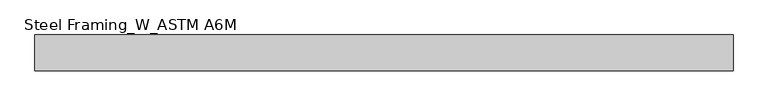
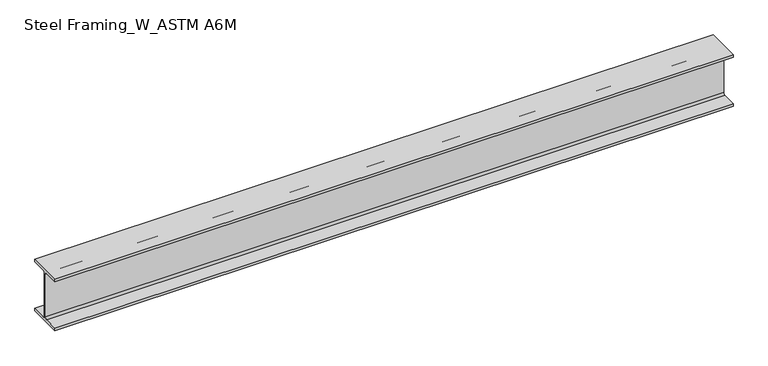
"""IFC4 building model written with IfcOpenShell, lengths in millimetres: beam geometry, Steel Framing_W_ASTM A6M : H_SB_AR_S02_W200x31.3_B6."""

from ifc_helpers import new_model, si_unit, point, frame, frame_2d, origin, place, context, project, spatial, polyline, circle_curve, trimmed, segment, composite_curve, outline, extrude, source, transform, mapped, element, save


def steel_framing_w_astm_a6m_88b43453(model_context):
    return source(origin(), model_context, "Body", "SweptSolid", [
        extrude(outline(composite_curve([segment(polyline([(67.0, -94.8), (67.0, -105.0), (-67.0, -105.0), (-67.0, -94.8), (-10.775, -94.8)]), True, "CONTINUOUS"), segment(trimmed(circle_curve(frame_2d((-10.775, -87.2)), 7.6), [point((-10.775, -94.8))], [point((-3.175, -87.2))], True, "CARTESIAN"), True, "CONTINUOUS"), segment(polyline([(-3.175, -87.2), (-3.175, 87.2)]), True, "CONTINUOUS"), segment(trimmed(circle_curve(frame_2d((-10.775, 87.2)), 7.6), [point((-3.175, 87.2))], [point((-10.775, 94.8))], True, "CARTESIAN"), True, "CONTINUOUS"), segment(polyline([(-10.775, 94.8), (-67.0, 94.8), (-67.0, 105.0), (67.0, 105.0), (67.0, 94.8), (10.775, 94.8)]), True, "CONTINUOUS"), segment(trimmed(circle_curve(frame_2d((10.775, 87.2)), 7.6), [point((10.775, 94.8))], [point((3.175, 87.2))], True, "CARTESIAN"), True, "CONTINUOUS"), segment(polyline([(3.175, 87.2), (3.175, -87.2)]), True, "CONTINUOUS"), segment(trimmed(circle_curve(frame_2d((10.775, -87.2)), 7.6), [point((3.175, -87.2))], [point((10.775, -94.8))], True, "CARTESIAN"), True, "CONTINUOUS"), segment(polyline([(10.775, -94.8), (67.0, -94.8)]), True, "CONTINUOUS")], self_intersect=False)), frame((-1274.5, 0.0, 0.0), z_axis=(1.0, 0.0, 0.0), x_axis=(0.0, 1.0, 0.0)), (0.0, 0.0, 1.0), 2620.8),
    ])


if __name__ == "__main__":
    model = new_model("IFC4")
    model_context = context("Model", 3, world=origin())
    ifc_project = project(units=[si_unit("LENGTHUNIT", "METRE", prefix="MILLI")], contexts=[model_context])
    site = spatial("IfcSite", under=ifc_project)
    building = spatial("IfcBuilding", under=site)
    placement = place(None, origin())
    steel_framing_w_astm_a6m_shape = steel_framing_w_astm_a6m_88b43453(model_context)
    element("IfcBeam", 1, ObjectType="Steel Framing_W_ASTM A6M : H_SB_AR_S02_W200x31.3_B6", at=placement, inside=building, context=model_context, shape_type="MappedRepresentation", body=[
        mapped(steel_framing_w_astm_a6m_shape, transform((0.0, 0.0, 0.0), x_axis=(1.0, 0.0, 0.0), y_axis=(0.0, 1.0, 0.0), z_axis=(0.0, 0.0, 1.0))),
    ])
    save(model, "model.ifc")

# Revit data of these elements
# Type "Steel Framing_W_ASTM A6M : H_SB_AR_S02_W200x31.3_B6"
#   Type Mark = "B6"
#   Section Name Key = "W8x21"
#   Width = 13.4 cm
#   Web Thickness = 0.635 cm
#   Web Fillet = 0.76 cm
#   Warping Constant = 40800.0 cm⁶
#   Torsional Moment of Inertia = 11.70 cm⁴
#   Section Area = 39.7 cm²
#   Plastic Modulus weak axis = 93.2 cm³
#   Plastic Modulus strong axis = 334.0 cm³
#   Perimeter = 0.93 m²/m
#   Nominal Weight = 31.30 kgf/m
#   Moment of Inertia weak axis = 407.00 cm⁴
#   Moment of Inertia strong axis = 3130.00 cm⁴
#   Height = 21.0 cm
#   Flange Thickness = 1.02 cm
#   Elastic Modulus weak axis = 60.8 cm³
#   Elastic Modulus strong axis = 298.0 cm³
#   Centroid Vertical = 10.5 cm
#   Centroid Horizontal = 6.7 cm
#   Length [instance default] = 1500 mm
#   Structural Material [instance default] = Steel, 45-345
#   Bolt Spacing = 0
#   Assembly Code = ""
# Element 1 (IfcBeam, "Steel Framing_W_ASTM A6M : H_SB_AR_S02_W200x31.3_B6")
#   Materials on its faces: "Steel, 45-345"
# Materials
#   "Steel, 45-345": class "Metal", colour RGB 189 187 185, transparency 0, Description = "Steel 345 MPa", Cost = 0
